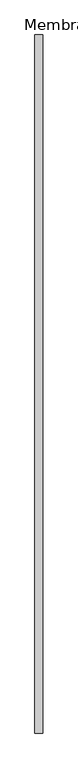
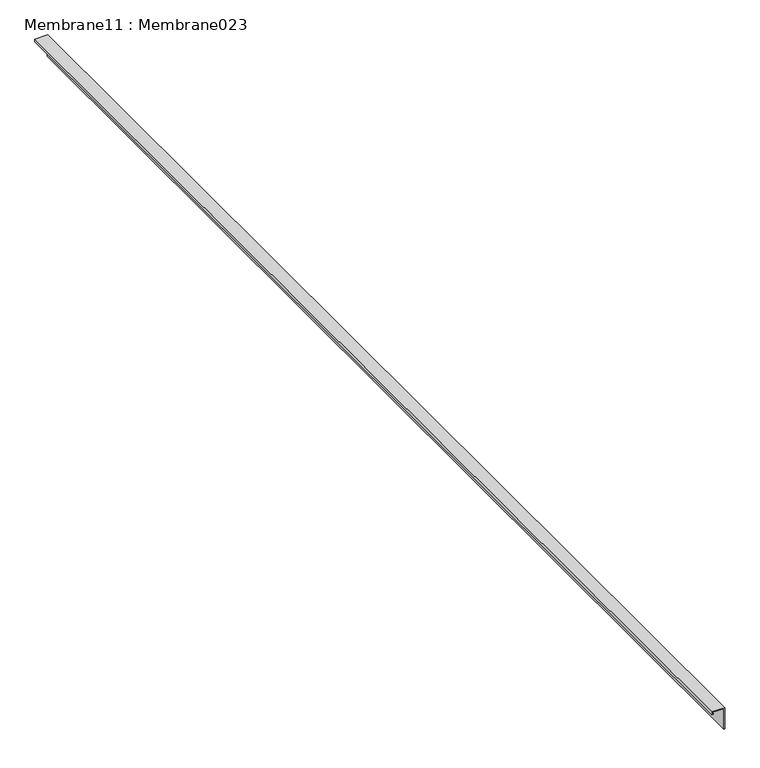
"""IFC4 building model written with IfcOpenShell, lengths in millimetres: proxy geometry, Membrane11 : Membrane023."""

from ifc_helpers import new_model, si_unit, frame, origin, place, context, project, spatial, polyline, outline, extrude, source, transform, mapped, element, save


def membrane11_membrane023_76801ec9(model_context):
    return source(origin(), model_context, "Body", "SweptSolid", [
        extrude(outline(polyline([(40164.2260083, -7231.852008), (40127.3960083, -7231.852008), (40127.3960083, -7230.582008), (40165.4960083, -7230.582008), (40165.4960083, -7252.807008), (40160.7462083, -7252.807008), (40160.7462083, -7249.8045516), (40162.0162083, -7249.8045516), (40162.0162083, -7251.537008), (40164.2260083, -7251.537008), (40164.2260083, -7231.852008)])), frame((0.0, 7182.1531721, 0.0), z_axis=(0.0, 1.0, 0.0), x_axis=(0.0, 0.0, 1.0)), (0.0, 0.0, 1.0), 2000.0),
    ])


if __name__ == "__main__":
    model = new_model("IFC4")
    model_context = context("Model", 3, world=origin())
    ifc_project = project(units=[si_unit("LENGTHUNIT", "METRE", prefix="MILLI")], contexts=[model_context])
    site = spatial("IfcSite", under=ifc_project)
    building = spatial("IfcBuilding", under=site)
    placement = place(None, origin())
    membrane11_membrane023_shape = membrane11_membrane023_76801ec9(model_context)
    element("IfcBuildingElementProxy", 1, Name="Membrane11 : Membrane023", ObjectType="Membrane11 : Membrane023", at=placement, inside=building, context=model_context, shape_type="MappedRepresentation", body=[
        mapped(membrane11_membrane023_shape, transform((0.0, 0.0, 0.0), x_axis=(1.0, 0.0, 0.0), y_axis=(0.0, 1.0, 0.0), z_axis=(0.0, 0.0, 1.0))),
    ])
    save(model, "model.ifc")

# Revit data of these elements
# Type "Membrane11 : Membrane023"
#   NameOverride = "Membrane023"
# Element 1 (IfcBuildingElementProxy, "Membrane11 : Membrane023")
#   Materials on its faces: "COPPER STUCCO J BEAD"
# Materials
#   "COPPER STUCCO J BEAD": class "Unassigned", colour RGB 251 232 155, transparency 0, Cost = 0
